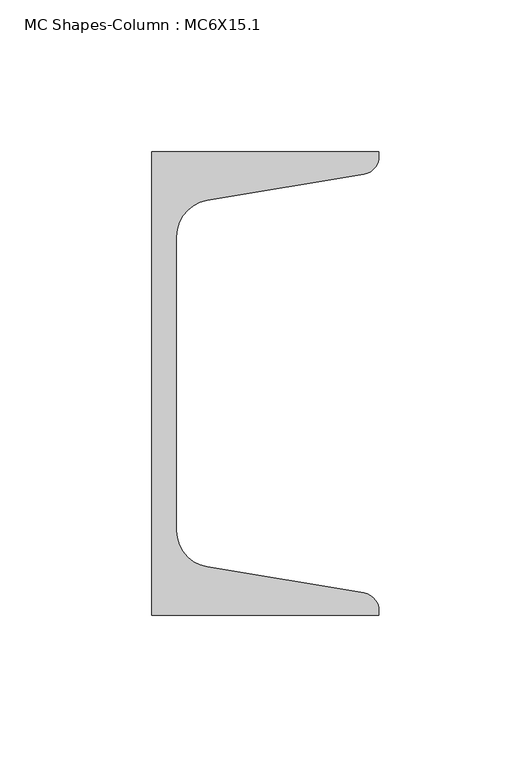
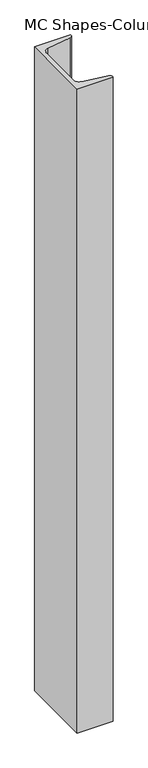
"""IFC4 building model written with IfcOpenShell, lengths in millimetres: column geometry, MC Shapes-Column : MC6X15.1."""

from ifc_helpers import new_model, si_unit, point, frame, frame_2d, origin, place, context, project, spatial, polyline, circle_curve, trimmed, segment, composite_curve, outline, extrude, source, transform, mapped, element, save


def mc_shapes_column_mc6x15_1_5d94ceb7(model_context):
    return source(origin(), model_context, "Body", "SweptSolid", [
        extrude(outline(composite_curve([segment(polyline([(-23.876, -76.2), (-23.876, 76.2), (50.8, 76.2), (50.8, 74.7994369)]), True, "CONTINUOUS"), segment(trimmed(circle_curve(frame_2d((44.7675, 74.7994369)), 6.0325), [point((50.8, 74.7994369))], [point((45.7592388, 68.8490159))], False, "CARTESIAN"), True, "CONTINUOUS"), segment(polyline([(45.7592388, 68.8490159), (-5.7680776, 60.2611126)]), True, "CONTINUOUS"), segment(trimmed(circle_curve(frame_2d((-3.7846, 48.3602706)), 12.065), [point((-5.7680776, 60.2611126))], [point((-15.8496, 48.3602706))], True, "CARTESIAN"), True, "CONTINUOUS"), segment(polyline([(-15.8496, 48.3602706), (-15.8496, -48.3602706)]), True, "CONTINUOUS"), segment(trimmed(circle_curve(frame_2d((-3.7846, -48.3602706)), 12.065), [point((-15.8496, -48.3602706))], [point((-5.7680776, -60.2611126))], True, "CARTESIAN"), True, "CONTINUOUS"), segment(polyline([(-5.7680776, -60.2611126), (45.7592388, -68.8490159)]), True, "CONTINUOUS"), segment(trimmed(circle_curve(frame_2d((44.7675, -74.7994369)), 6.0325), [point((45.7592388, -68.8490159))], [point((50.8, -74.7994369))], False, "CARTESIAN"), True, "CONTINUOUS"), segment(polyline([(50.8, -74.7994369), (50.8, -76.2), (-23.876, -76.2)]), True, "CONTINUOUS")], self_intersect=False)), frame((0.0, 0.0, 4610.1), z_axis=(0.0, 0.0, 1.0), x_axis=(1.0, 0.0, 0.0)), (0.0, 0.0, 1.0), 1409.7),
    ])


if __name__ == "__main__":
    model = new_model("IFC4")
    model_context = context("Model", 3, world=origin())
    ifc_project = project(units=[si_unit("LENGTHUNIT", "METRE", prefix="MILLI")], contexts=[model_context])
    site = spatial("IfcSite", under=ifc_project)
    building = spatial("IfcBuilding", under=site)
    placement = place(None, origin())
    mc_shapes_column_mc6x15_1_shape = mc_shapes_column_mc6x15_1_5d94ceb7(model_context)
    element("IfcColumn", 1, ObjectType="MC Shapes-Column : MC6X15.1", at=placement, inside=building, context=model_context, shape_type="MappedRepresentation", body=[
        mapped(mc_shapes_column_mc6x15_1_shape, transform((0.0, 0.0, 0.0), x_axis=(1.0, 0.0, 0.0), y_axis=(0.0, 1.0, 0.0), z_axis=(0.0, 0.0, 1.0))),
    ])
    save(model, "model.ifc")

# Revit data of these elements
# Type "MC Shapes-Column : MC6X15.1"
#   Section Name Key = "MC6X15.1"
#   Assembly Code = "B10"
#   Width = 2.940"
#   Web Thickness = 0.316"
#   Web Fillet = 0.475"
#   Warping Constant = 20.50 in⁶
#   Torsional Moment of Inertia = 0.285 in⁴
#   Sloped Flange Angle = 9.46234°
#   Section Area = 4.44 in²
#   Plastic Modulus weak axis = 3.30 in³
#   Plastic Modulus strong axis = 9.83 in³
#   Nominal Weight = 15.10 lbf/ft
#   Moment of Inertia weak axis = 3.46 in⁴
#   Moment of Inertia strong axis = 24.90 in⁴
#   Height = 6.000"
#   Flange Thickness Location = 1.312"
#   Flange Thickness = 0.475"
#   Flange Fillet = 0.2375"
#   Elastic Modulus weak axis = 1.73 in³
#   Elastic Modulus strong axis = 8.30 in³
#   Centroid Vertical = 3.000"
#   Centroid Horizontal = 0.940"
#   Bolt Spacing = 0' - 1 3/4"
#   Structural Material [instance default] = Steel ASTM A36
#   Principal Axes Angle = 0
# Element 1 (IfcColumn, "MC Shapes-Column : MC6X15.1")
#   Structural Material = Metal - Steel - ASTM A992
#   Materials on its faces: "Metal - Steel - ASTM A992"
# Materials
#   "Steel ASTM A36": class "Metal", colour RGB 199 199 199, transparency 0, Description = "Structural steel, ASTM A36 Grade B, mill finish", Cost = 0
#   "Metal - Steel - ASTM A992": class "Metal", colour RGB 255 128 0, transparency 0
